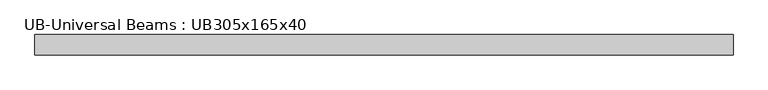
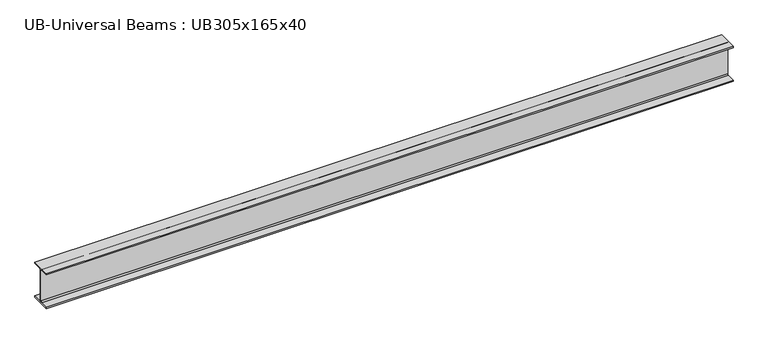
"""IFC4 building model written with IfcOpenShell, lengths in millimetres: beam geometry, UB-Universal Beams : UB305x165x40."""

from ifc_helpers import new_model, si_unit, point, frame, frame_2d, origin, place, context, project, spatial, polyline, circle_curve, trimmed, segment, composite_curve, outline, extrude, source, transform, mapped, element, save


def ub_universal_beams_ub305x165x40_d3799931(model_context):
    return source(origin(), model_context, "Body", "SweptSolid", [
        extrude(outline(composite_curve([segment(polyline([(82.5, -141.5), (82.5, -151.7), (-82.5, -151.7), (-82.5, -141.5), (-11.9, -141.5)]), True, "CONTINUOUS"), segment(trimmed(circle_curve(frame_2d((-11.9, -132.6)), 8.9), [point((-11.9, -141.5))], [point((-3.0, -132.6))], True, "CARTESIAN"), True, "CONTINUOUS"), segment(polyline([(-3.0, -132.6), (-3.0, 132.6)]), True, "CONTINUOUS"), segment(trimmed(circle_curve(frame_2d((-11.9, 132.6)), 8.9), [point((-3.0, 132.6))], [point((-11.9, 141.5))], True, "CARTESIAN"), True, "CONTINUOUS"), segment(polyline([(-11.9, 141.5), (-82.5, 141.5), (-82.5, 151.7), (82.5, 151.7), (82.5, 141.5), (11.9, 141.5)]), True, "CONTINUOUS"), segment(trimmed(circle_curve(frame_2d((11.9, 132.6)), 8.9), [point((11.9, 141.5))], [point((3.0, 132.6))], True, "CARTESIAN"), True, "CONTINUOUS"), segment(polyline([(3.0, 132.6), (3.0, -132.6)]), True, "CONTINUOUS"), segment(trimmed(circle_curve(frame_2d((11.9, -132.6)), 8.9), [point((3.0, -132.6))], [point((11.9, -141.5))], True, "CARTESIAN"), True, "CONTINUOUS"), segment(polyline([(11.9, -141.5), (82.5, -141.5)]), True, "CONTINUOUS")], self_intersect=False)), frame((-2828.4, 0.0, 0.0), z_axis=(1.0, 0.0, 0.0), x_axis=(0.0, 1.0, 0.0)), (0.0, 0.0, 1.0), 5656.8),
    ])


if __name__ == "__main__":
    model = new_model("IFC4")
    model_context = context("Model", 3, world=origin())
    ifc_project = project(units=[si_unit("LENGTHUNIT", "METRE", prefix="MILLI")], contexts=[model_context])
    site = spatial("IfcSite", under=ifc_project)
    building = spatial("IfcBuilding", under=site)
    placement = place(None, origin())
    ub_universal_beams_ub305x165x40_shape = ub_universal_beams_ub305x165x40_d3799931(model_context)
    element("IfcBeam", 1, ObjectType="UB-Universal Beams : UB305x165x40", at=placement, inside=building, context=model_context, shape_type="MappedRepresentation", body=[
        mapped(ub_universal_beams_ub305x165x40_shape, transform((0.0, 0.0, 0.0), x_axis=(1.0, 0.0, 0.0), y_axis=(0.0, 1.0, 0.0), z_axis=(0.0, 0.0, 1.0))),
    ])
    save(model, "model.ifc")

# Revit data of these elements
# Type "UB-Universal Beams : UB305x165x40"
#   Section Name Key = "UB305X165X40"
#   Width = 16.5 cm
#   Web Thickness = 0.6 cm
#   Web Fillet = 0.89 cm
#   Warping Constant = 164000.0 cm⁶
#   Torsional Moment of Inertia = 14.70 cm⁴
#   Section Area = 51.3 cm²
#   Plastic Modulus weak axis = 142.0 cm³
#   Plastic Modulus strong axis = 623.0 cm³
#   Nominal Weight = 40.2999 kgf/m
#   Moment of Inertia weak axis = 764.00 cm⁴
#   Moment of Inertia strong axis = 8503.00 cm⁴
#   Height = 30.34 cm
#   Flange Thickness = 1.02 cm
#   Elastic Modulus weak axis = 92.6 cm³
#   Elastic Modulus strong axis = 560.0 cm³
#   Centroid Vertical = 15.17 cm
#   Centroid Horizontal = 8.25 cm
#   Bolt Spacing = 9.0 cm
#   Length [instance default] = 1500 mm
#   Structural Material [instance default] = Metal - Steel 43-275
#   Type Comments = ""
#   Assembly Code = ""
# Element 1 (IfcBeam, "UB-Universal Beams : UB305x165x40")
#   Materials on its faces: "Metal - Steel 43-275"
# Materials
#   "Metal - Steel 43-275": class "Metal", colour RGB 247 247 247, transparency 0, Cost = 0
